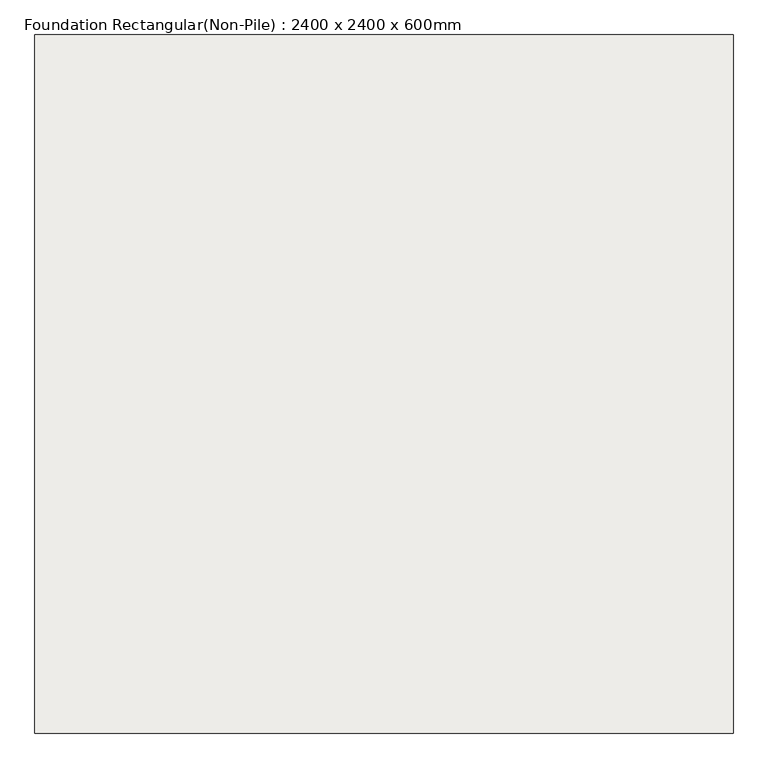
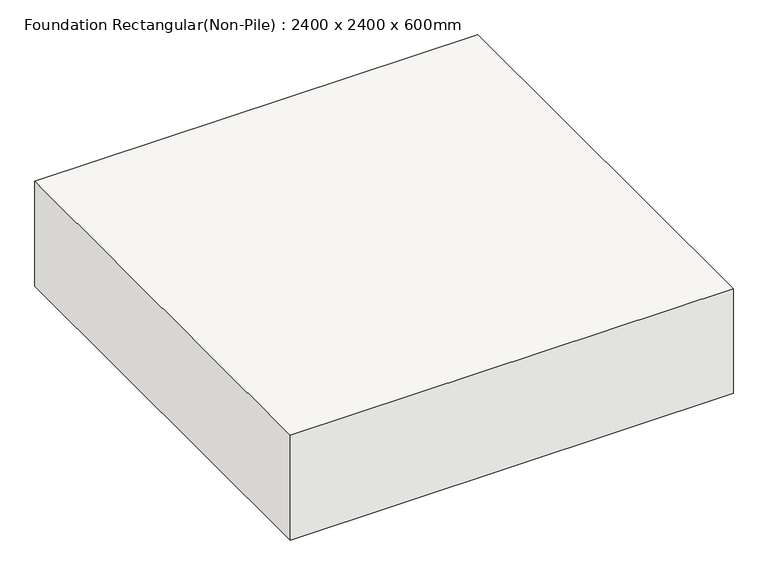
"""IFC4 building model written with IfcOpenShell, lengths in millimetres: slab geometry, Foundation Rectangular(Non-Pile) : 2400 x 2400 x 600mm."""

from ifc_helpers import new_model, si_unit, frame, origin, place, context, project, spatial, polyline, outline, extrude, source, transform, mapped, element, save


def foundation_rectangular_non_pile_2400_x_2400_x_600mm_9fdc1d6b(model_context):
    return source(origin(), model_context, "Body", "SweptSolid", [
        extrude(outline(polyline([(1200.0, 1200.0), (1200.0, -1200.0), (-1200.0, -1200.0), (-1200.0, 1200.0), (1200.0, 1200.0)])), frame((0.0, 0.0, -600.0), z_axis=(0.0, 0.0, 1.0), x_axis=(1.0, 0.0, 0.0)), (0.0, 0.0, 1.0), 600.0),
    ])


if __name__ == "__main__":
    model = new_model("IFC4")
    model_context = context("Model", 3, world=origin())
    ifc_project = project(units=[si_unit("LENGTHUNIT", "METRE", prefix="MILLI")], contexts=[model_context])
    site = spatial("IfcSite", under=ifc_project)
    building = spatial("IfcBuilding", under=site)
    placement = place(None, origin())
    foundation_rectangular_non_pile_2400_x_2400_x_600mm_shape = foundation_rectangular_non_pile_2400_x_2400_x_600mm_9fdc1d6b(model_context)
    element("IfcSlab", 1, ObjectType="Foundation Rectangular(Non-Pile) : 2400 x 2400 x 600mm", at=placement, inside=building, context=model_context, shape_type="MappedRepresentation", body=[
        mapped(foundation_rectangular_non_pile_2400_x_2400_x_600mm_shape, transform((0.0, 0.0, 0.0), x_axis=(1.0, 0.0, 0.0), y_axis=(0.0, 1.0, 0.0), z_axis=(0.0, 0.0, 1.0))),
    ])
    save(model, "model.ifc")

# Revit data of these elements
# Type "Foundation Rectangular(Non-Pile) : 2400 x 2400 x 600mm"
#   Width = 2400 mm
#   Length = 2400 mm
#   Foundation Thickness = 600 mm
#   Structural Material [instance default] = 콘크리트 - 현장타설 콘크리트
#   Assembly Code = ""
# Element 1 (IfcSlab, "Foundation Rectangular(Non-Pile) : 2400 x 2400 x 600mm")
#   Materials on its faces: "콘크리트 - 현장타설 콘크리트"
# Materials
#   "콘크리트 - 현장타설 콘크리트": class "콘크리트", colour RGB 192 192 192, transparency 0, Cost = 0
